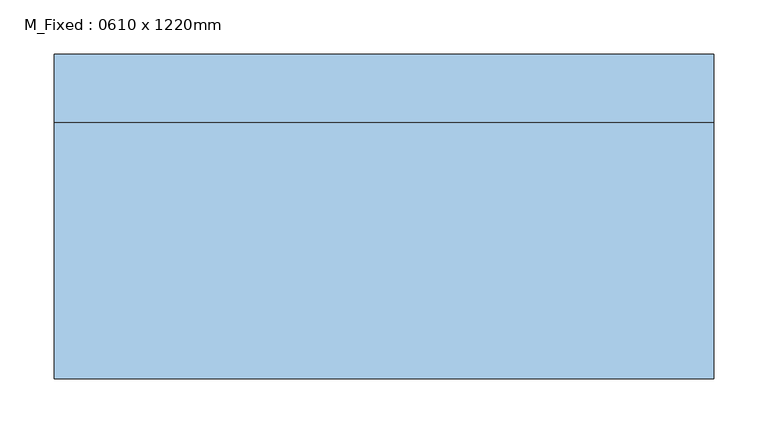
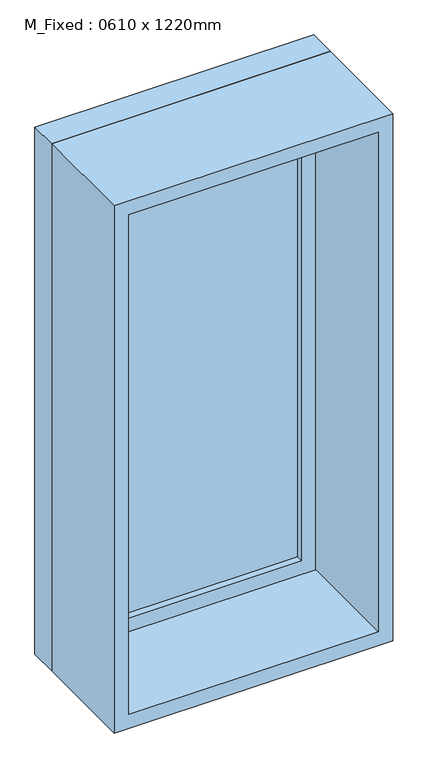
"""IFC4 building model written with IfcOpenShell, lengths in millimetres: window geometry, M_Fixed : 0610 x 1220mm."""

from ifc_helpers import new_model, si_unit, frame, origin, place, context, project, spatial, polyline, outline, extrude, source, transform, mapped, element, save


def m_fixed_0610_x_1220mm_961092c7(model_context):
    return source(origin(), model_context, "Body", "SweptSolid", [
        extrude(outline(polyline([(-242.0, 128.0), (242.0, 128.0), (242.0, 116.0), (-242.0, 116.0), (-242.0, 128.0)])), frame((0.0, 0.0, 978.0), z_axis=(0.0, 0.0, 1.0), x_axis=(1.0, 0.0, 0.0)), (0.0, 0.0, 1.0), 1094.0),
        extrude(outline(polyline([(2116.0, -286.0), (934.0, -286.0), (934.0, 286.0), (2116.0, 286.0), (2116.0, -286.0)]), holes=[polyline([(2072.0, -242.0), (2072.0, 242.0), (978.0, 242.0), (978.0, -242.0), (2072.0, -242.0)])]), frame((0.0, 100.0, 0.0), z_axis=(0.0, 1.0, 0.0), x_axis=(0.0, 0.0, 1.0)), (0.0, 0.0, 1.0), 44.0),
        extrude(outline(polyline([(2135.0, -305.0), (915.0, -305.0), (915.0, 305.0), (2135.0, 305.0), (2135.0, -305.0)]), holes=[polyline([(2116.0, -286.0), (2116.0, 286.0), (934.0, 286.0), (934.0, -286.0), (2116.0, -286.0)])]), frame((0.0, 100.0, 0.0), z_axis=(0.0, 1.0, 0.0), x_axis=(0.0, 0.0, 1.0)), (0.0, 0.0, 1.0), 63.0),
        extrude(outline(polyline([(2135.0, -305.0), (915.0, -305.0), (915.0, 305.0), (2135.0, 305.0), (2135.0, -305.0)]), holes=[polyline([(2103.0, -273.0), (2103.0, 273.0), (947.0, 273.0), (947.0, -273.0), (2103.0, -273.0)])]), frame((0.0, -137.0, 0.0), z_axis=(0.0, 1.0, 0.0), x_axis=(0.0, 0.0, 1.0)), (0.0, 0.0, 1.0), 237.0),
    ])


if __name__ == "__main__":
    model = new_model("IFC4")
    model_context = context("Model", 3, world=origin())
    ifc_project = project(units=[si_unit("LENGTHUNIT", "METRE", prefix="MILLI")], contexts=[model_context])
    site = spatial("IfcSite", under=ifc_project)
    building = spatial("IfcBuilding", under=site)
    placement = place(None, origin())
    m_fixed_0610_x_1220mm_shape = m_fixed_0610_x_1220mm_961092c7(model_context)
    element("IfcWindow", 1, ObjectType="M_Fixed : 0610 x 1220mm", at=placement, inside=building, context=model_context, shape_type="MappedRepresentation", body=[
        mapped(m_fixed_0610_x_1220mm_shape, transform((0.0, 0.0, 0.0), x_axis=(1.0, 0.0, 0.0), y_axis=(0.0, 1.0, 0.0), z_axis=(0.0, 0.0, 1.0))),
    ])
    save(model, "model.ifc")

# Revit data of these elements
# Type "M_Fixed : 0610 x 1220mm"
#   Type Mark = "13"
#   Construction Type Id = "GSP4R"
#   Analytic Construction = "1/8 in Pilkington single glazing"
#   Visual Light Transmittance = 0.9
#   Thermal Resistance (R) = 0.271106 (m²·K)/W
#   Solar Heat Gain Coefficient = 0.78
#   Heat Transfer Coefficient (U) = 3.6886 W/(m²·K)
#   Height = 1220 mm
#   Default Sill Height = 915 mm
#   Width = 610 mm
#   Window Inset = 19 mm
#   Define Thermal Properties by = 1
#   Frame Exterior Material = Sash
#   Frame Interior Material = Sash
#   Glass Pane Material = Glass
#   Sash = Sash
#   Wall Closure = (empty or 0)
# Element 1 (IfcWindow, "M_Fixed : 0610 x 1220mm")
#   Materials on its faces: "Sash", "Glass"
# Materials
#   "Sash": class "Wood", colour RGB 224 178 126, transparency 0, Cost = 0
#   "Glass": class "Glass", colour RGB 0 128 192, transparency 0.75, Description = "Soda Lime Glass", Cost = 0
